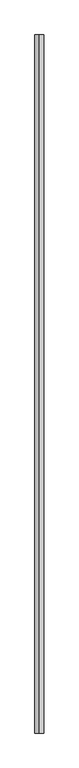
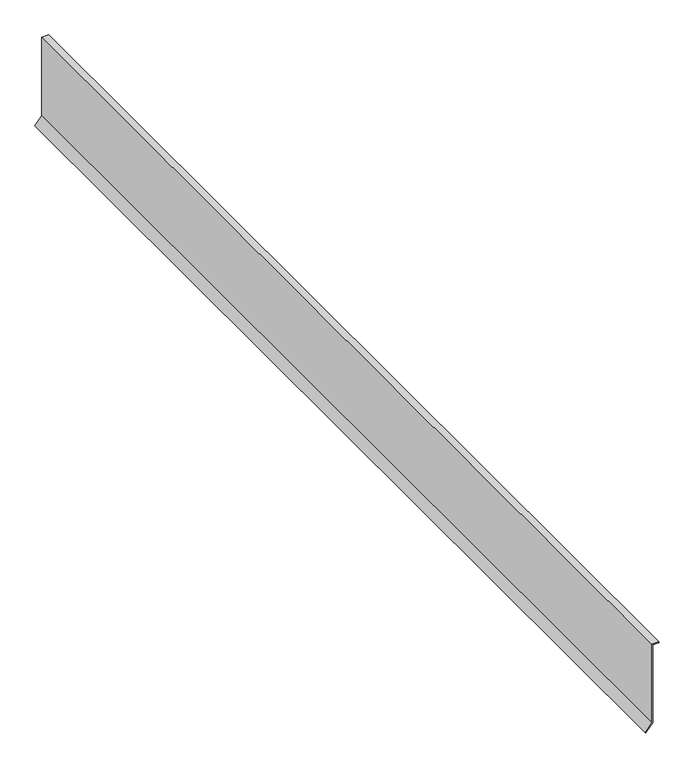
"""IFC4 building model written with IfcOpenShell, lengths in millimetres: proxy geometry, GRAVEL STOP003 3744 : GRAVEL STOP003 3744."""

from ifc_helpers import new_model, si_unit, frame, origin, place, context, project, spatial, polyline, outline, extrude, source, transform, mapped, element, save


def generic_models_73d50619(model_context):
    return source(origin(), model_context, "Body", "SweptSolid", [
        extrude(outline(polyline([(40082.2407116, -5046.164524), (40081.3605882, -5045.0615204), (40097.4918556, -5032.189842), (40253.3245993, -5032.189842), (40253.3245993, -5020.4219233), (40254.7357103, -5020.4219233), (40254.7357103, -5033.600953), (40097.9858473, -5033.600953), (40082.2407116, -5046.164524)])), frame((0.0, -1052.8906573, 0.0), z_axis=(0.0, 1.0, 0.0), x_axis=(0.0, 0.0, 1.0)), (0.0, 0.0, 1.0), 2000.25),
    ])


if __name__ == "__main__":
    model = new_model("IFC4")
    model_context = context("Model", 3, world=origin())
    ifc_project = project(units=[si_unit("LENGTHUNIT", "METRE", prefix="MILLI")], contexts=[model_context])
    site = spatial("IfcSite", under=ifc_project)
    building = spatial("IfcBuilding", under=site)
    placement = place(None, origin())
    generic_models_shape = generic_models_73d50619(model_context)
    element("IfcBuildingElementProxy", 1, Name="GRAVEL STOP003 3744 : GRAVEL STOP003 3744", ObjectType="GRAVEL STOP003 3744 : GRAVEL STOP003 3744", at=placement, inside=building, context=model_context, shape_type="MappedRepresentation", body=[
        mapped(generic_models_shape, transform((0.0, 0.0, 0.0), x_axis=(1.0, 0.0, 0.0), y_axis=(0.0, 1.0, 0.0), z_axis=(0.0, 0.0, 1.0))),
    ])
    save(model, "model.ifc")

# Revit data of these elements
# Type "GRAVEL STOP003 3744 : GRAVEL STOP003 3744"
#   NameOverride = "GRAVEL STOP003"
# Element 1 (IfcBuildingElementProxy, "GRAVEL STOP003 3744 : GRAVEL STOP003 3744")
#   Materials on its faces: "GRAVEL STOP REQUIRED WITH GRAVEL SURFACE SYSTEMS"
# Materials
#   "GRAVEL STOP REQUIRED WITH GRAVEL SURFACE SYSTEMS": class "Unassigned", colour RGB 170 170 127, transparency 0
